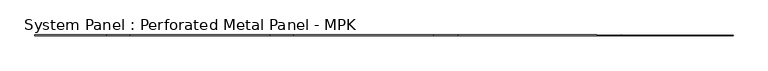
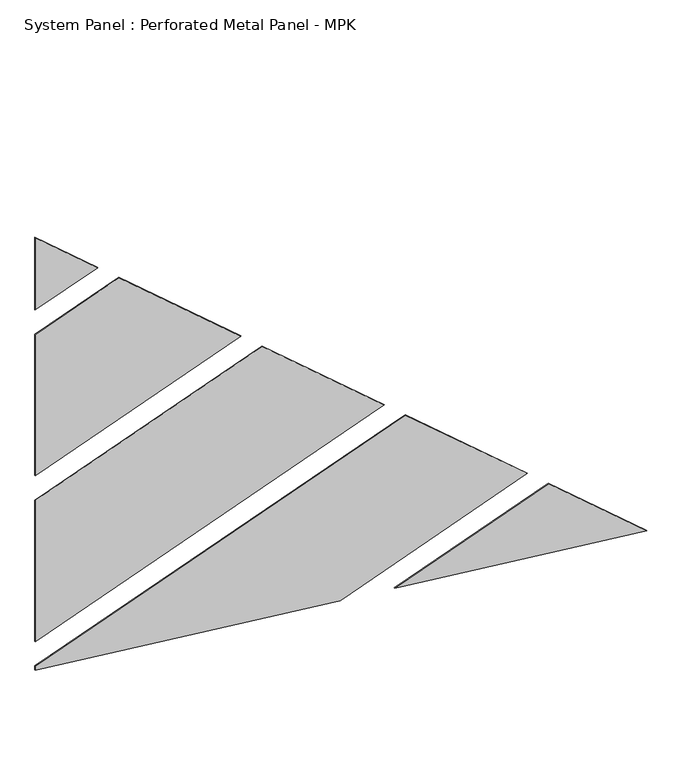
"""IFC4 building model written with IfcOpenShell, lengths in millimetres: plate geometry, System Panel : Perforated Metal Panel - MPK."""

from ifc_helpers import new_model, si_unit, frame, origin, place, context, project, spatial, polyline, outline, extrude, source, transform, mapped, element, save


def system_panel_perforated_metal_panel_mpk_a5ab8e0f(model_context):
    return source(origin(), model_context, "Body", "SweptSolid", [
        extrude(outline(polyline([(16602.3536102, -11346.7703881), (17453.084874, -9029.7329419), (19437.6967847, -11346.7703881), (16602.3536102, -11346.7703881)])), frame((0.0, 0.0, 0.0), z_axis=(0.0, 1.0, 0.0), x_axis=(0.0, 0.0, 1.0)), (0.0, 0.0, 1.0), 20.0),
        extrude(outline(polyline([(10096.7032471, -11346.7703881), (12899.4240285, -3713.3269281), (16778.3914363, -8242.0273197), (15638.4435263, -11346.7703881), (10096.7032471, -11346.7703881)])), frame((0.0, 0.0, 0.0), z_axis=(0.0, 1.0, 0.0), x_axis=(0.0, 0.0, 1.0)), (0.0, 0.0, 1.0), 20.0),
        extrude(outline(polyline([(3591.0528839, -11346.7703881), (8345.7631829, 1603.0790857), (12224.7305908, -2925.6213059), (9132.7931631, -11346.7703881), (3591.0528839, -11346.7703881)])), frame((0.0, 0.0, 0.0), z_axis=(0.0, 1.0, 0.0), x_axis=(0.0, 0.0, 1.0)), (0.0, 0.0, 1.0), 20.0),
        extrude(outline(polyline([(2474.3752228, -11346.7703881), (1240.4694871, -30.0994692), (3792.1023373, 6919.4850995), (7671.0697452, 2390.7847079), (2627.1427999, -11346.7703881), (2474.3752228, -11346.7703881)])), frame((0.0, 0.0, 0.0), z_axis=(0.0, 1.0, 0.0), x_axis=(0.0, 0.0, 1.0)), (0.0, 0.0, 1.0), 20.0),
        extrude(outline(polyline([(1019.7643088, 1994.0809857), (0.0, 11346.7703881), (3117.4088996, 7707.1907217), (1019.7643088, 1994.0809857)])), frame((0.0, 0.0, 0.0), z_axis=(0.0, 1.0, 0.0), x_axis=(0.0, 0.0, 1.0)), (0.0, 0.0, 1.0), 20.0),
    ])


if __name__ == "__main__":
    model = new_model("IFC4")
    model_context = context("Model", 3, world=origin())
    ifc_project = project(units=[si_unit("LENGTHUNIT", "METRE", prefix="MILLI")], contexts=[model_context])
    site = spatial("IfcSite", under=ifc_project)
    building = spatial("IfcBuilding", under=site)
    placement = place(None, origin())
    system_panel_perforated_metal_panel_mpk_shape = system_panel_perforated_metal_panel_mpk_a5ab8e0f(model_context)
    element("IfcPlate", 1, ObjectType="System Panel : Perforated Metal Panel - MPK", at=placement, inside=building, context=model_context, shape_type="MappedRepresentation", body=[
        mapped(system_panel_perforated_metal_panel_mpk_shape, transform((0.0, 0.0, 0.0), x_axis=(1.0, 0.0, 0.0), y_axis=(0.0, 1.0, 0.0), z_axis=(0.0, 0.0, 1.0))),
    ])
    save(model, "model.ifc")

# Revit data of these elements
# Element 1 (IfcPlate, "System Panel : Perforated Metal Panel - MPK")
#   Materials on its faces: "Perforated  Metal Panels - MPK"
# Materials
#   "Perforated  Metal Panels - MPK": class "Miscellaneous", colour RGB 127 127 127, transparency 0
